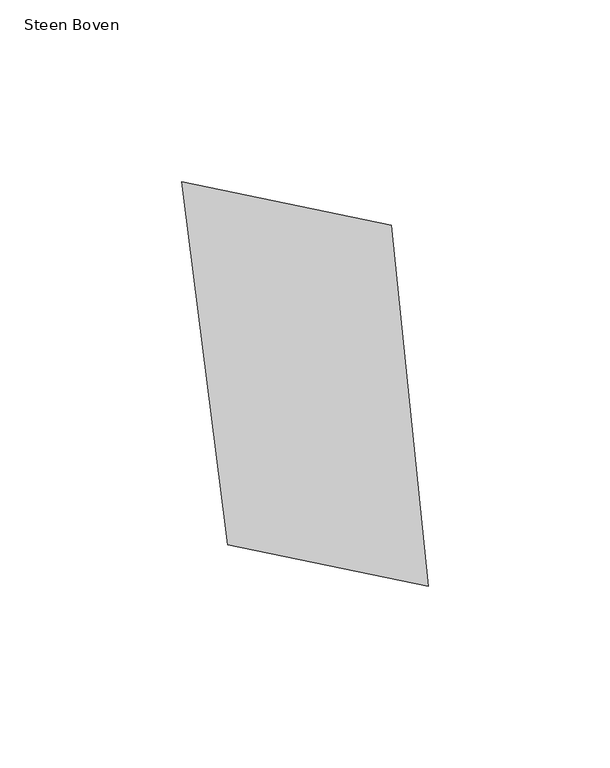
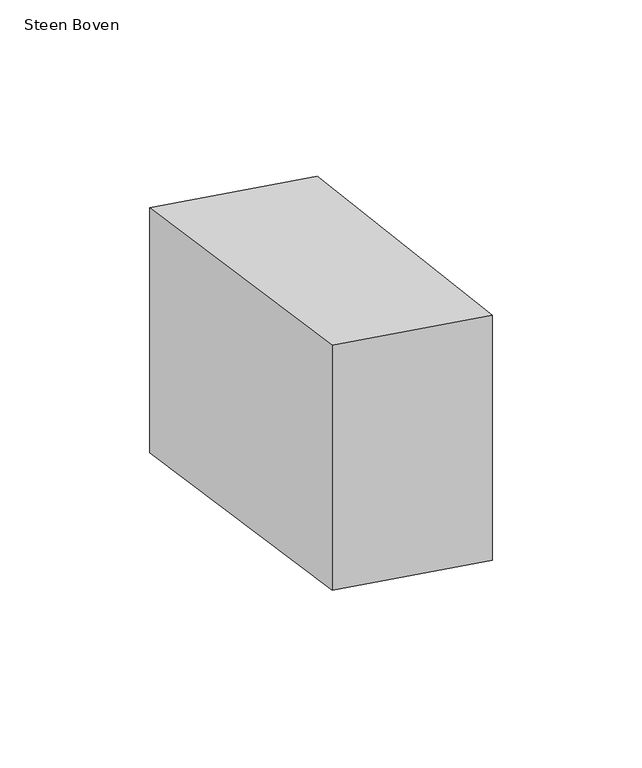
"""IFC4 building model written with IfcOpenShell, lengths in millimetres: proxy geometry, 00_GMA_steen_versie_4 : Steen Boven."""

from ifc_helpers import new_model, si_unit, origin, origin_with_axes, place, context, project, spatial, polyline, outline, extrude, source, transform, mapped, element, save


def steen_boven_c095d349(model_context):
    return source(origin(), model_context, "Body", "SweptSolid", [
        extrude(outline(polyline([(95.3421463, 121.8030811), (105.4675319, 22.4031643), (50.3229905, 33.8737991), (37.6194207, 133.8454716), (95.3421463, 121.8030811)])), origin_with_axes(), (0.0, 0.0, 1.0), 100.0),
    ])


if __name__ == "__main__":
    model = new_model("IFC4")
    model_context = context("Model", 3, world=origin())
    ifc_project = project(units=[si_unit("LENGTHUNIT", "METRE", prefix="MILLI")], contexts=[model_context])
    site = spatial("IfcSite", under=ifc_project)
    building = spatial("IfcBuilding", under=site)
    placement = place(None, origin())
    steen_boven_shape = steen_boven_c095d349(model_context)
    element("IfcBuildingElementProxy", 1, Name="00_GMA_steen_versie_4 : Steen Boven", ObjectType="00_GMA_steen_versie_4 : Steen Boven", at=placement, inside=building, context=model_context, shape_type="MappedRepresentation", body=[
        mapped(steen_boven_shape, transform((0.0, 0.0, 0.0), x_axis=(1.0, 0.0, 0.0), y_axis=(0.0, 1.0, 0.0), z_axis=(0.0, 0.0, 1.0))),
    ])
    save(model, "model.ifc")

# Revit data of these elements
# Type "00_GMA_steen_versie_4 : Steen Boven"
#   StootVoegHalfBoven [instance default] = 5 mm
#   StootVoegHalf [instance default] = 5 mm
#   StootVoegBreedteOnder = 10 mm
#   StootVoegBreedteBoven = 10 mm
#   Steendikte = 100 mm
#   LintVoegOnderHalf = 5 mm
#   LintVoegOnder = 10 mm
#   LintVoegBovenHalf = 0 mm
#   LintVoegBoven = 0 mm
#   materiaal = none
#   MateriaalVoeg = none
#   Default Elevation = 0
